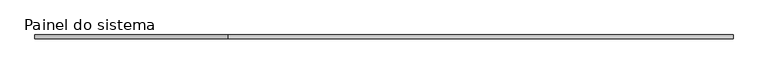
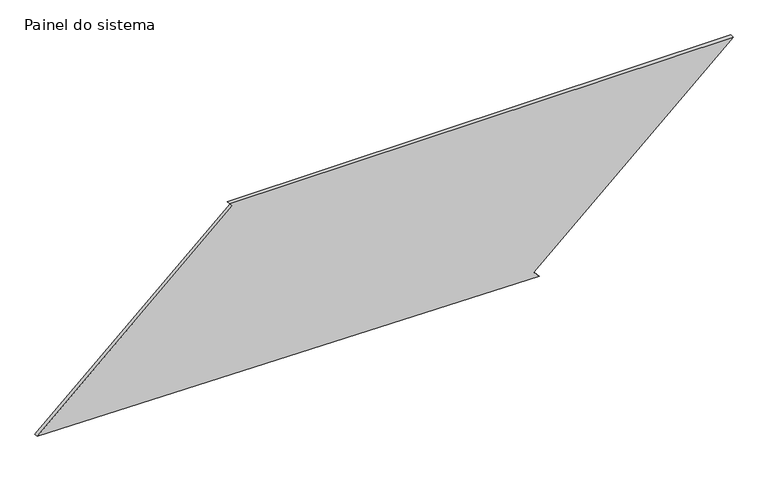
"""IFC4 building model written with IfcOpenShell, lengths in millimetres: plate geometry, Painel do sistema : Envidraçado."""

from ifc_helpers import new_model, si_unit, frame, origin, place, context, project, spatial, polyline, outline, extrude, source, transform, mapped, element, save


def painel_do_sistema_677b8234(model_context):
    return source(origin(), model_context, "Body", "SweptSolid", [
        extrude(outline(polyline([(0.0, 956.1751339), (37.1936933, 922.759132), (1147.313368, 2158.3782472), (1147.313368, -964.1606224), (1128.7165214, -947.4526215), (40.7822662, -2158.3782472), (0.0, 956.1751339)])), frame((0.0, 24.5, 0.0), z_axis=(0.0, 1.0, 0.0), x_axis=(0.0, 0.0, 1.0)), (0.0, 0.0, 1.0), 25.0),
    ])


if __name__ == "__main__":
    model = new_model("IFC4")
    model_context = context("Model", 3, world=origin())
    ifc_project = project(units=[si_unit("LENGTHUNIT", "METRE", prefix="MILLI")], contexts=[model_context])
    site = spatial("IfcSite", under=ifc_project)
    building = spatial("IfcBuilding", under=site)
    placement = place(None, origin())
    painel_do_sistema_shape = painel_do_sistema_677b8234(model_context)
    element("IfcPlate", 1, ObjectType="Painel do sistema : Envidraçado", at=placement, inside=building, context=model_context, shape_type="MappedRepresentation", body=[
        mapped(painel_do_sistema_shape, transform((0.0, 0.0, 0.0), x_axis=(1.0, 0.0, 0.0), y_axis=(0.0, 1.0, 0.0), z_axis=(0.0, 0.0, 1.0))),
    ])
    save(model, "model.ifc")

# Revit data of these elements
# Type "Painel do sistema : Envidraçado"
#   Construction Type Id = "GSP4R"
#   Analytic Construction = "Vidraça única Pilkington 1/8 pol"
#   Visual Light Transmittance = 0.9
#   Solar Heat Gain Coefficient = 0.86
#   Heat Transfer Coefficient (U) = 6.7069 W/(m²·K)
# Element 1 (IfcPlate, "Painel do sistema : Envidraçado")
#   Materials on its faces: "Vidro"
# Materials
#   "Vidro": class "Vidro", colour RGB 0 128 192, transparency 0.9, Description = "Vidro de sílica", Cost = 0
